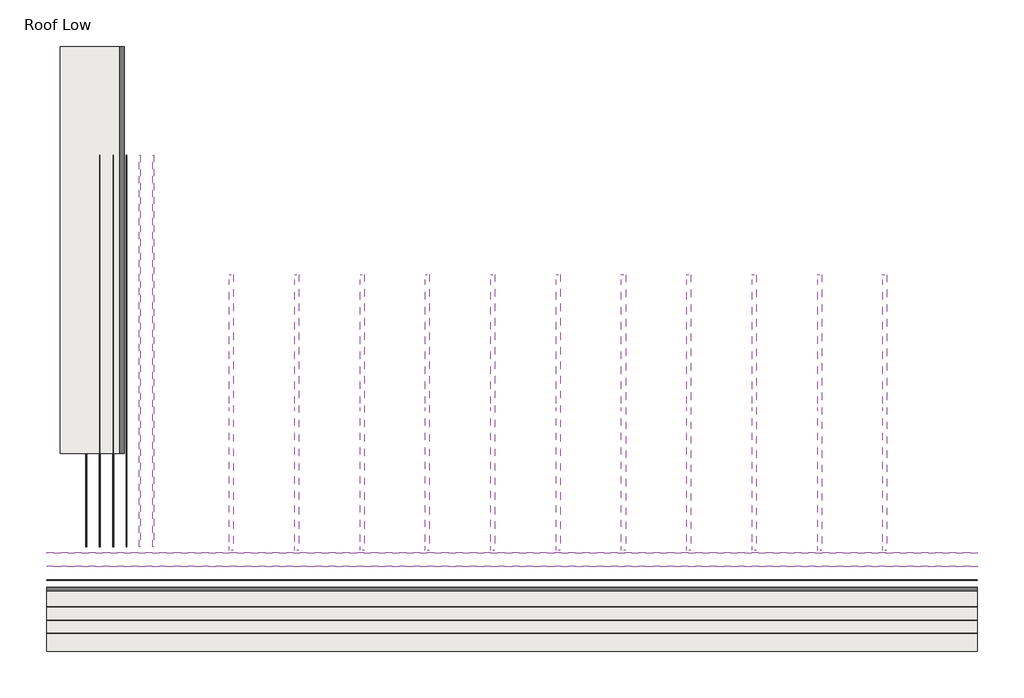
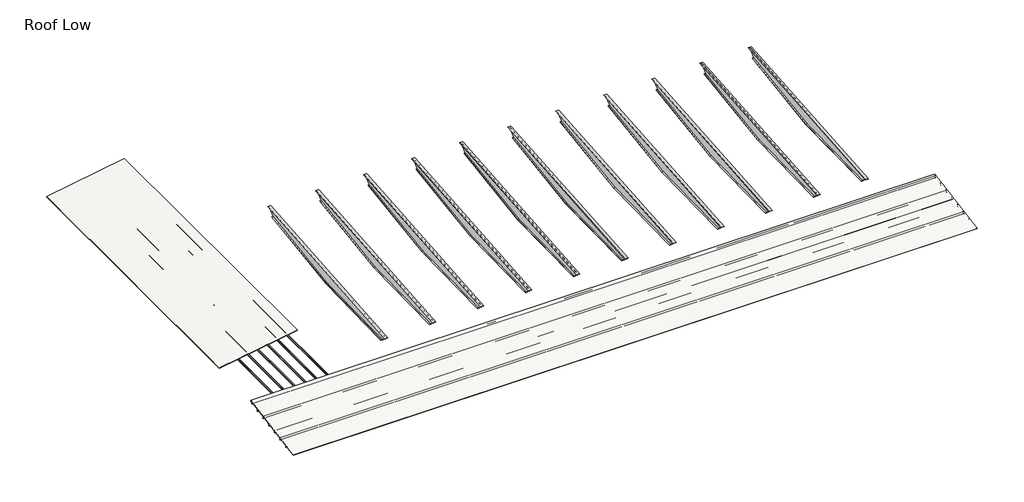
# One storey: 24 beams, 2 roofs.
"""IFC4 building model written with IfcOpenShell, lengths in millimetres."""

import ifcopenshell
import ifcopenshell.guid

model = None  # the IFC model being written
_history = None  # IfcOwnerHistory: only IFC2X3 demands one
_inside = {}  # id of a spatial element -> (the spatial element, [elements in it])
_under = {}  # id of a project, library or spatial element -> (it, [spatial elements below it])
_declared = {}  # id of a project -> (the project, [libraries it declares])
_typed = {}  # id of a type object -> (the type object, [elements of that type])
_made_of = {}  # id of a material, layer set ... -> (it, [elements and type objects made of it])


def new_model(schema):
    """Start an empty IFC model of exactly this schema.

    Asked for "IFC4X3", IfcOpenShell would pick the latest addendum, in which some entities
    have other attributes; the version numbers below select the first issue.
    IFC2X3 requires an IfcOwnerHistory on every rooted entity: one is made here for all.
    """
    global model, _history
    if schema == "IFC4X3":
        model = ifcopenshell.file(schema_version=(4, 3, 0, 0))
    else:
        model = ifcopenshell.file(schema=schema)
    _inside.clear()
    _under.clear()
    _declared.clear()
    _typed.clear()
    _made_of.clear()
    _history = None
    if model.schema == "IFC2X3":
        org = make("IfcOrganization", Name="unknown")
        user = make(
            "IfcPersonAndOrganization",
            ThePerson=make("IfcPerson", FamilyName="unknown"),
            TheOrganization=org,
        )
        app = make(
            "IfcApplication",
            ApplicationDeveloper=org,
            Version="unknown",
            ApplicationFullName="unknown",
            ApplicationIdentifier="unknown",
        )
        _history = make(
            "IfcOwnerHistory",
            OwningUser=user,
            OwningApplication=app,
            ChangeAction="ADDED",
            CreationDate=0,
        )
    return model


def make(cls, **values):
    """One entity of the class cls with the attributes given. An attribute that is None is left unset."""
    return model.create_entity(
        cls, **{name: value for name, value in values.items() if value is not None}
    )


def rooted(cls, **values):
    """An entity with a GlobalId (a new one), such as an element, a storey or a relation."""
    return make(cls, GlobalId=ifcopenshell.guid.new(), OwnerHistory=_history, **values)


def si_unit(unit_type, name, prefix=None):
    """IfcSIUnit, for example si_unit("LENGTHUNIT", "METRE", prefix="MILLI")."""
    return make("IfcSIUnit", UnitType=unit_type, Prefix=prefix, Name=name)


def assignment(units):
    """IfcUnitAssignment: the units of a project."""
    return None if units is None else make("IfcUnitAssignment", Units=units)


def point(xyz):
    """IfcCartesianPoint."""
    return None if xyz is None else make("IfcCartesianPoint", Coordinates=xyz)


def direction(xyz):
    """IfcDirection."""
    return None if xyz is None else make("IfcDirection", DirectionRatios=xyz)


def frame(location, z_axis=None, x_axis=None):
    """IfcAxis2Placement3D, a coordinate frame: its origin and axes. An axis left out is left unset."""
    return make(
        "IfcAxis2Placement3D",
        Location=point(location),
        Axis=direction(z_axis),
        RefDirection=direction(x_axis),
    )


def frame_2d(location, x_axis=None):
    """IfcAxis2Placement2D, a coordinate frame in the plane: its origin and x axis."""
    return make(
        "IfcAxis2Placement2D", Location=point(location), RefDirection=direction(x_axis)
    )


def origin():
    """The frame at (0, 0, 0) with its axes left unset."""
    return frame((0.0, 0.0, 0.0))


def place(relative_to, where):
    """IfcLocalPlacement: puts the frame where relative to a parent placement (None: the world)."""
    return make(
        "IfcLocalPlacement", PlacementRelTo=relative_to, RelativePlacement=where
    )


def context(
    kind, dimensions, precision=None, world=None, true_north=None, identifier=None
):
    """IfcGeometricRepresentationContext, for example the 3D "Model" context."""
    return make(
        "IfcGeometricRepresentationContext",
        ContextIdentifier=identifier,
        ContextType=kind,
        CoordinateSpaceDimension=dimensions,
        Precision=precision,
        WorldCoordinateSystem=world,
        TrueNorth=true_north,
    )


def project(units=None, contexts=None):
    """IfcProject with its units and contexts."""
    return rooted(
        "IfcProject",
        Name="project",
        RepresentationContexts=contexts,
        UnitsInContext=assignment(units),
    )


def spatial(cls, under=None, at=None, **own):
    """A site, building, storey or space (cls), placed at a placement, below another one or the project."""
    s = rooted(cls, ObjectPlacement=at, **own)
    if under is not None:
        _under.setdefault(under.id(), (under, []))[1].append(s)
    return s


def polyline(points):
    """IfcPolyline through the points."""
    return make("IfcPolyline", Points=[point(p) for p in points])


def circle_curve(where, radius):
    """IfcCircle in the frame where."""
    return make("IfcCircle", Position=where, Radius=radius)


def trimmed(basis, trim1, trim2, sense, master):
    """IfcTrimmedCurve: the piece of a basis curve between two trims."""
    return make(
        "IfcTrimmedCurve",
        BasisCurve=basis,
        Trim1=trim1,
        Trim2=trim2,
        SenseAgreement=sense,
        MasterRepresentation=master,
    )


def segment(curve, same_sense, transition):
    """IfcCompositeCurveSegment."""
    return make(
        "IfcCompositeCurveSegment",
        Transition=transition,
        SameSense=same_sense,
        ParentCurve=curve,
    )


def composite_curve(segments, self_intersect=None):
    """IfcCompositeCurve: segments joined end to end."""
    return make("IfcCompositeCurve", Segments=segments, SelfIntersect=self_intersect)


def outline(outer, holes=None, kind="AREA"):
    """IfcArbitraryClosedProfileDef: a profile drawn as a closed curve; with holes, ...WithVoids."""
    if holes is None:
        return make("IfcArbitraryClosedProfileDef", ProfileType=kind, OuterCurve=outer)
    return make(
        "IfcArbitraryProfileDefWithVoids",
        ProfileType=kind,
        OuterCurve=outer,
        InnerCurves=holes,
    )


def extrude(swept, where, along, depth):
    """IfcExtrudedAreaSolid: the profile swept, set in the frame where, extruded along a direction by depth."""
    return make(
        "IfcExtrudedAreaSolid",
        SweptArea=swept,
        Position=where,
        ExtrudedDirection=direction(along),
        Depth=depth,
    )


def shape(context_of_items, identifier, shape_type, items):
    """IfcShapeRepresentation: the items that make up one representation, for example the "Body"."""
    return make(
        "IfcShapeRepresentation",
        ContextOfItems=context_of_items,
        RepresentationIdentifier=identifier,
        RepresentationType=shape_type,
        Items=items,
    )


def source(mapping_origin, context_of_items, identifier, shape_type, items):
    """IfcRepresentationMap: a shape defined once, which mapped items show again and again."""
    return make(
        "IfcRepresentationMap",
        MappingOrigin=mapping_origin,
        MappedRepresentation=shape(context_of_items, identifier, shape_type, items),
    )


def transform(
    local_origin,
    x_axis=None,
    y_axis=None,
    z_axis=None,
    scale=None,
    scale2=None,
    scale3=None,
    uniform=True,
):
    """IfcCartesianTransformationOperator3D, or its non-uniform kind. x_axis, y_axis, z_axis: its Axis1, 2, 3."""
    if uniform:
        return make(
            "IfcCartesianTransformationOperator3D",
            Axis1=direction(x_axis),
            Axis2=direction(y_axis),
            LocalOrigin=point(local_origin),
            Scale=scale,
            Axis3=direction(z_axis),
        )
    return make(
        "IfcCartesianTransformationOperator3DnonUniform",
        Axis1=direction(x_axis),
        Axis2=direction(y_axis),
        LocalOrigin=point(local_origin),
        Scale=scale,
        Axis3=direction(z_axis),
        Scale2=scale2,
        Scale3=scale3,
    )


def mapped(mapping_source, mapping_target):
    """IfcMappedItem: shows the shape of a source again, moved by a transform."""
    return make(
        "IfcMappedItem", MappingSource=mapping_source, MappingTarget=mapping_target
    )


def made_of(thing, what):
    """Note that an element or type object is made of a material, layer set ...; save() writes the relation."""
    if what is not None:
        _made_of.setdefault(what.id(), (what, []))[1].append(thing)
    return thing


def element(
    cls,
    number,
    at=None,
    inside=None,
    cuts=None,
    type_object=None,
    material=None,
    context=None,
    identifier="Body",
    shape_type=None,
    held_by="IfcProductDefinitionShape",
    body=None,
    shapes=None,
    **own,
):
    """One element of the class cls, such as IfcWall. Its Tag is "e" and its number.

    at: its placement. inside: the storey or other place that contains it. cuts: it is an
    opening in that element (IfcRelVoidsElement). A single representation is given by context,
    identifier, shape_type and body (its items); several are given by shapes. held_by: the class
    of the entity that holds the representations. save() writes the other relations.
    """
    e = rooted(cls, Tag="e%d" % number, ObjectPlacement=at, **own)
    if body is not None:
        shapes = [shape(context, identifier, shape_type, body)]
    if shapes is not None:
        e.Representation = make(held_by, Representations=shapes)
    if inside is not None:
        _inside.setdefault(inside.id(), (inside, []))[1].append(e)
    if cuts is not None:
        rooted(
            "IfcRelVoidsElement", RelatingBuildingElement=cuts, RelatedOpeningElement=e
        )
    if type_object is not None:
        _typed.setdefault(type_object.id(), (type_object, []))[1].append(e)
    return made_of(e, material)


def aggregate(whole, parts):
    """IfcRelAggregates: a whole, such as a stair, and the parts it consists of."""
    return rooted("IfcRelAggregates", RelatingObject=whole, RelatedObjects=parts)


def save(model, path):
    """Write the relations noted so far, then the file.

    IfcRelAggregates (storeys below a building ...), IfcRelContainedInSpatialStructure (elements
    in a storey), IfcRelDefinesByType, IfcRelAssociatesMaterial and IfcRelDeclares: one each for
    every whole, place, type object, material and project.
    """
    for whole, parts in _under.values():
        aggregate(whole, parts)
    for where, things in _inside.values():
        rooted(
            "IfcRelContainedInSpatialStructure",
            RelatedElements=things,
            RelatingStructure=where,
        )
    for kind, things in _typed.values():
        rooted("IfcRelDefinesByType", RelatedObjects=things, RelatingType=kind)
    for what, things in _made_of.values():
        rooted("IfcRelAssociatesMaterial", RelatedObjects=things, RelatingMaterial=what)
    for by, libraries in _declared.values():
        rooted("IfcRelDeclares", RelatingContext=by, RelatedDefinitions=libraries)
    model.write(path)


def family7_family7_14774666(model_context):
    return source(origin(), model_context, "Body", "SweptSolid", [
        extrude(outline(polyline([(-914.4, -14659.3825135), (-1828.8, 0.0), (-914.4, 14336.786696), (-31.75, 15508.1028078), (-31.75, -15542.0325135), (-914.4, -14659.3825135)])), frame((0.0, -15.875, 0.0), z_axis=(0.0, 1.0, 0.0), x_axis=(0.0, 0.0, 1.0)), (0.0, 0.0, 1.0), 31.75),
        extrude(outline(polyline([(-914.4, 14336.786696), (-1828.8, 0.0), (-914.4, -14659.3825135), (-948.3280154, -14625.4544981), (-1860.6130939, 0.0222371), (-949.1562421, 14290.6636049), (-914.4, 14336.786696)])), frame((0.0, -228.6, 0.0), z_axis=(0.0, 1.0, 0.0), x_axis=(0.0, 0.0, 1.0)), (0.0, 0.0, 1.0), 457.2),
        extrude(outline(polyline([(-31.75, 15508.1028078), (0.0, 15550.2364809), (0.0, -15573.7825135), (-31.75, -15542.0325135), (-31.75, 15508.1028078)])), frame((0.0, -228.6, 0.0), z_axis=(0.0, 1.0, 0.0), x_axis=(0.0, 0.0, 1.0)), (0.0, 0.0, 1.0), 457.2),
    ])


def beam_6747da0e(model_context):
    return source(origin(), model_context, "Body", "SweptSolid", [
        extrude(outline(composite_curve([segment(polyline([(63.5, 127.0), (75.745104, 112.4068534), (73.6169367, 110.621109), (62.204539, 124.221875), (3.3005807, 124.221875)]), True, "CONTINUOUS"), segment(trimmed(circle_curve(frame_2d((3.3741066, 122.2381931)), 1.9850441), [point((3.3005807, 124.221875))], [point((1.3890625, 122.2381931))], True, "CARTESIAN"), True, "CONTINUOUS"), segment(polyline([(1.3890625, 122.2381931), (1.3890625, -122.2375)]), True, "CONTINUOUS"), segment(trimmed(circle_curve(frame_2d((-3.3734375, -122.2375)), 4.7625), [point((1.3890625, -122.2375))], [point((-3.3734375, -127.0))], False, "CARTESIAN"), True, "CONTINUOUS"), segment(polyline([(-3.3734375, -127.0), (-63.5, -127.0), (-75.745104, -112.4068534), (-73.6169367, -110.621109), (-62.204539, -124.221875), (-3.2694106, -124.221875)]), True, "CONTINUOUS"), segment(trimmed(circle_curve(frame_2d((-3.3748024, -122.2389339)), 1.9857399), [point((-3.2694106, -124.221875))], [point((-1.3890625, -122.2389339))], True, "CARTESIAN"), True, "CONTINUOUS"), segment(polyline([(-1.3890625, -122.2389339), (-1.3890625, 122.2375)]), True, "CONTINUOUS"), segment(trimmed(circle_curve(frame_2d((3.3734375, 122.2375)), 4.7625), [point((-1.3890625, 122.2375))], [point((3.3734375, 127.0))], False, "CARTESIAN"), True, "CONTINUOUS"), segment(polyline([(3.3734375, 127.0), (63.5, 127.0)]), True, "CONTINUOUS")], self_intersect=False)), frame((-52273.2, 0.0, 0.0), z_axis=(1.0, 0.0, 0.0), x_axis=(0.0, 1.0, 0.0)), (0.0, 0.0, 1.0), 104546.4),
    ])


def beam_884d35ae(model_context):
    return source(origin(), model_context, "Body", "SweptSolid", [
        extrude(outline(composite_curve([segment(polyline([(63.5, 127.0), (75.745104, 112.4068534), (73.6169367, 110.621109), (62.204539, 124.221875), (3.3005807, 124.221875)]), True, "CONTINUOUS"), segment(trimmed(circle_curve(frame_2d((3.3741066, 122.2381931)), 1.9850441), [point((3.3005807, 124.221875))], [point((1.3890625, 122.2381931))], True, "CARTESIAN"), True, "CONTINUOUS"), segment(polyline([(1.3890625, 122.2381931), (1.3890625, -122.2375)]), True, "CONTINUOUS"), segment(trimmed(circle_curve(frame_2d((-3.3734375, -122.2375)), 4.7625), [point((1.3890625, -122.2375))], [point((-3.3734375, -127.0))], False, "CARTESIAN"), True, "CONTINUOUS"), segment(polyline([(-3.3734375, -127.0), (-63.5, -127.0), (-75.745104, -112.4068534), (-73.6169367, -110.621109), (-62.204539, -124.221875), (-3.2694106, -124.221875)]), True, "CONTINUOUS"), segment(trimmed(circle_curve(frame_2d((-3.3748024, -122.2389339)), 1.9857399), [point((-3.2694106, -124.221875))], [point((-1.3890625, -122.2389339))], True, "CARTESIAN"), True, "CONTINUOUS"), segment(polyline([(-1.3890625, -122.2389339), (-1.3890625, 122.2375)]), True, "CONTINUOUS"), segment(trimmed(circle_curve(frame_2d((3.3734375, 122.2375)), 4.7625), [point((-1.3890625, 122.2375))], [point((3.3734375, 127.0))], False, "CARTESIAN"), True, "CONTINUOUS"), segment(polyline([(3.3734375, 127.0), (63.5, 127.0)]), True, "CONTINUOUS")], self_intersect=False)), frame((-22098.0, 0.0, 0.0), z_axis=(1.0, 0.0, 0.0), x_axis=(0.0, 1.0, 0.0)), (0.0, 0.0, 1.0), 44025.82),
    ])


model = new_model("IFC4")

# Units and contexts
model_context = context("Model", 3, world=origin())
ifc_project = project(units=[si_unit("LENGTHUNIT", "METRE", prefix="MILLI")], contexts=[model_context])

# Site, building, storey
site = spatial("IfcSite", under=ifc_project)
building = spatial("IfcBuilding", under=site)
storey = spatial("IfcBuildingStorey", under=building, Name="Roof Low", Elevation=3657.6)

# Beams
placement = place(None, origin())
family7_family7_shape = family7_family7_14774666(model_context)
element("IfcBeam", 1, ObjectType="Family7 : Family7", at=placement, inside=storey, context=model_context, shape_type="MappedRepresentation", body=[
    mapped(family7_family7_shape, transform((586368.9117241, -552426.8407337, 9726.0083875), x_axis=(1.32038933737171e-12, 0.9965457582448788, 0.08304547985374926), y_axis=(-1.0, 1.316111794066913e-12, 0.0), z_axis=(0.0, -0.08304547985374934, 0.9965457582448789))),
])
element("IfcBeam", 2, ObjectType="Family7 : Family7", at=placement, inside=storey, context=model_context, shape_type="MappedRepresentation", body=[
    mapped(family7_family7_shape, transform((593709.5117241, -552426.8407337, 9726.0083875), x_axis=(1.3203893373716879e-12, 0.9965457582448789, 0.08304547985374928), y_axis=(-1.0, 1.3161117940668907e-12, 0.0), z_axis=(0.0, -0.08304547985374937, 0.9965457582448789))),
])
element("IfcBeam", 3, ObjectType="Family7 : Family7", at=placement, inside=storey, context=model_context, shape_type="MappedRepresentation", body=[
    mapped(family7_family7_shape, transform((601050.1117241, -552426.8407337, 9726.0083875), x_axis=(1.3203893373716624e-12, 0.9965457582448789, 0.08304547985374897), y_axis=(-1.0, 1.3161117940668655e-12, 0.0), z_axis=(0.0, -0.08304547985374904, 0.9965457582448789))),
])
element("IfcBeam", 4, ObjectType="Family7 : Family7", at=placement, inside=storey, context=model_context, shape_type="MappedRepresentation", body=[
    mapped(family7_family7_shape, transform((608390.7117241, -552426.8407337, 9726.0083875), x_axis=(1.3203893373716398e-12, 0.9965457582448789, 0.0830454798537492), y_axis=(-1.0, 1.3161117940668428e-12, 0.0), z_axis=(0.0, -0.08304547985374928, 0.9965457582448789))),
])
element("IfcBeam", 5, ObjectType="Family7 : Family7", at=placement, inside=storey, context=model_context, shape_type="MappedRepresentation", body=[
    mapped(family7_family7_shape, transform((615731.3117241, -552426.8407337, 9726.0083875), x_axis=(1.3203893373716176e-12, 0.9965457582448789, 0.08304547985374894), y_axis=(-1.0, 1.3161117940668206e-12, 0.0), z_axis=(0.0, -0.08304547985374901, 0.9965457582448789))),
])
element("IfcBeam", 6, ObjectType="Family7 : Family7", at=placement, inside=storey, context=model_context, shape_type="MappedRepresentation", body=[
    mapped(family7_family7_shape, transform((623071.9117241, -552426.8407337, 9726.0083875), x_axis=(1.3203893373715917e-12, 0.9965457582448788, 0.0830454798537492), y_axis=(-1.0, 1.316111794066795e-12, 0.0), z_axis=(0.0, -0.0830454798537493, 0.9965457582448789))),
])
element("IfcBeam", 7, ObjectType="Family7 : Family7", at=placement, inside=storey, context=model_context, shape_type="MappedRepresentation", body=[
    mapped(family7_family7_shape, transform((630412.5117241, -552426.8407337, 9726.0083875), x_axis=(1.3179754628973985e-12, 0.9965457582448789, 0.08304547985374894), y_axis=(-1.0, 1.3137062576986022e-12, 0.0), z_axis=(0.0, -0.08304547985374901, 0.9965457582448789))),
])
element("IfcBeam", 8, ObjectType="Family7 : Family7", at=placement, inside=storey, context=model_context, shape_type="MappedRepresentation", body=[
    mapped(family7_family7_shape, transform((637753.1117241, -552426.8407337, 9726.0083875), x_axis=(1.317975462897376e-12, 0.9965457582448789, 0.08304547985374888), y_axis=(-1.0, 1.3137062576985798e-12, 0.0), z_axis=(0.0, -0.08304547985374897, 0.9965457582448789))),
])
element("IfcBeam", 9, ObjectType="Family7 : Family7", at=placement, inside=storey, context=model_context, shape_type="MappedRepresentation", body=[
    mapped(family7_family7_shape, transform((645093.7117241, -552426.8407337, 9726.0083875), x_axis=(1.3179754628973506e-12, 0.996545758244879, 0.08304547985374865), y_axis=(-1.0, 1.3137062576985543e-12, 0.0), z_axis=(0.0, -0.08304547985374879, 0.9965457582448789))),
])
element("IfcBeam", 10, ObjectType="Family7 : Family7", at=placement, inside=storey, context=model_context, shape_type="MappedRepresentation", body=[
    mapped(family7_family7_shape, transform((652434.3117241, -552426.8407337, 9726.0083875), x_axis=(1.317975462897328e-12, 0.9965457582448788, 0.08304547985374917), y_axis=(-1.0, 1.313706257698532e-12, 0.0), z_axis=(0.0, -0.08304547985374927, 0.9965457582448789))),
])
element("IfcBeam", 11, ObjectType="Family7 : Family7", at=placement, inside=storey, context=model_context, shape_type="MappedRepresentation", body=[
    mapped(family7_family7_shape, transform((659774.9117241, -552426.8407337, 9726.0083875), x_axis=(1.3179754628973058e-12, 0.9965457582448788, 0.08304547985374891), y_axis=(-0.9999999999999999, 1.3137062576985097e-12, 0.0), z_axis=(0.0, -0.083045479853749, 0.9965457582448789))),
])
beam_shape = beam_6747da0e(model_context)
element("IfcBeam", 12, ObjectType="Girt_Z : 10\"D", at=placement, inside=storey, context=model_context, shape_type="MappedRepresentation", body=[
    mapped(beam_shape, transform((617890.3117239, -568231.6177833, 5372.7057404), x_axis=(1.0, 0.0, 0.0), y_axis=(0.0, 0.9863939238321444, 0.16439898730535388), z_axis=(0.0, -0.16439898730535388, 0.9863939238321444))),
])
element("IfcBeam", 13, ObjectType="Girt_Z : 10\"D", at=placement, inside=storey, context=model_context, shape_type="MappedRepresentation", body=[
    mapped(beam_shape, transform((617890.3117239, -569734.8821232, 5122.1616837), x_axis=(1.0, 0.0, 0.0), y_axis=(0.0, 0.9863939238321444, 0.16439898730535388), z_axis=(0.0, -0.16439898730535388, 0.9863939238321444))),
])
element("IfcBeam", 14, ObjectType="Girt_Z : 10\"D", at=placement, inside=storey, context=model_context, shape_type="MappedRepresentation", body=[
    mapped(beam_shape, transform((617890.3117239, -571238.1464631, 4871.6176271), x_axis=(1.0, 0.0, 0.0), y_axis=(0.0, 0.9863939238321444, 0.16439898730535388), z_axis=(0.0, -0.16439898730535388, 0.9863939238321444))),
])
element("IfcBeam", 15, ObjectType="Girt_Z : 10\"D", at=placement, inside=storey, context=model_context, shape_type="MappedRepresentation", body=[
    mapped(beam_shape, transform((617890.3117239, -572741.410803, 4621.0735704), x_axis=(1.0, 0.0, 0.0), y_axis=(0.0, 0.9863939238321444, 0.16439898730535388), z_axis=(0.0, -0.16439898730535388, 0.9863939238321444))),
])
element("IfcBeam", 16, ObjectType="Girt_Z : 10\"D", at=placement, inside=storey, context=model_context, shape_type="MappedRepresentation", body=[
    mapped(beam_shape, transform((617890.3117239, -574244.6751429, 4370.5295137), x_axis=(1.0, 0.0, 0.0), y_axis=(0.0, 0.9863939238321444, 0.16439898730535388), z_axis=(0.0, -0.16439898730535388, 0.9863939238321444))),
])
element("IfcBeam", 17, ObjectType="Girt_Z : 10\"D", at=placement, inside=storey, context=model_context, shape_type="MappedRepresentation", body=[
    mapped(beam_shape, transform((617890.3117239, -575747.9394829, 4119.9854571), x_axis=(1.0, 0.0, 0.0), y_axis=(0.0, 0.9863939238321444, 0.16439898730535388), z_axis=(0.0, -0.16439898730535388, 0.9863939238321444))),
])
element("IfcBeam", 18, ObjectType="Girt_Z : 10\"D", at=placement, inside=storey, context=model_context, shape_type="MappedRepresentation", body=[
    mapped(beam_shape, transform((617890.3117239, -577251.2038228, 3869.4414004), x_axis=(1.0, 0.0, 0.0), y_axis=(0.0, 0.9863939238321444, 0.16439898730535388), z_axis=(0.0, -0.16439898730535388, 0.9863939238321444))),
])
beam_2_shape = beam_884d35ae(model_context)
element("IfcBeam", 19, ObjectType="Girt_Z : 10\"D", at=placement, inside=storey, context=model_context, shape_type="MappedRepresentation", body=[
    mapped(beam_2_shape, transform((577613.4981197, -545593.3413841, 5277.7495395), x_axis=(0.0, -1.0, 0.0), y_axis=(0.986393923832142, 0.0, 0.16439898730536787), z_axis=(-0.16439898730536787, 0.0, 0.986393923832142))),
])
element("IfcBeam", 20, ObjectType="Girt_Z : 10\"D", at=placement, inside=storey, context=model_context, shape_type="MappedRepresentation", body=[
    mapped(beam_2_shape, transform((576110.2337798, -545593.3413841, 5027.2054829), x_axis=(0.0, -1.0, 0.0), y_axis=(0.986393923832142, 0.0, 0.16439898730536787), z_axis=(-0.16439898730536787, 0.0, 0.986393923832142))),
])
element("IfcBeam", 21, ObjectType="Girt_Z : 10\"D", at=placement, inside=storey, context=model_context, shape_type="MappedRepresentation", body=[
    mapped(beam_2_shape, transform((574606.9694399, -545593.3413841, 4776.6614262), x_axis=(0.0, -1.0, 0.0), y_axis=(0.986393923832142, 0.0, 0.16439898730536787), z_axis=(-0.16439898730536787, 0.0, 0.986393923832142))),
])
element("IfcBeam", 22, ObjectType="Girt_Z : 10\"D", at=placement, inside=storey, context=model_context, shape_type="MappedRepresentation", body=[
    mapped(beam_2_shape, transform((573103.7050999, -545593.3413841, 4526.1173696), x_axis=(0.0, -1.0, 0.0), y_axis=(0.986393923832142, 0.0, 0.16439898730536787), z_axis=(-0.16439898730536787, 0.0, 0.986393923832142))),
])
element("IfcBeam", 23, ObjectType="Girt_Z : 10\"D", at=placement, inside=storey, context=model_context, shape_type="MappedRepresentation", body=[
    mapped(beam_2_shape, transform((571600.44076, -545593.3413841, 4275.5733129), x_axis=(0.0, -1.0, 0.0), y_axis=(0.986393923832142, 0.0, 0.16439898730536787), z_axis=(-0.16439898730536787, 0.0, 0.986393923832142))),
])
element("IfcBeam", 24, ObjectType="Girt_Z : 10\"D", at=placement, inside=storey, context=model_context, shape_type="MappedRepresentation", body=[
    mapped(beam_2_shape, transform((570097.1764201, -545593.3413841, 4025.0292563), x_axis=(0.0, -1.0, 0.0), y_axis=(0.986393923832142, 0.0, 0.16439898730536787), z_axis=(-0.16439898730536787, 0.0, 0.986393923832142))),
])

# Roofs
element("IfcRoof", 25, ObjectType="Roof_High", at=placement, inside=storey, context=model_context, shape_type="SweptSolid", body=[
    extrude(outline(polyline([(-579273.7413841, 3738.3546979), (-567945.3413841, 5626.4213646), (-567945.3413841, 5549.1702804), (-579273.7413841, 3661.1036138), (-579273.7413841, 3738.3546979)])), frame((565617.1117239, 0.0, 0.0), z_axis=(1.0, 0.0, 0.0), x_axis=(0.0, 1.0, 0.0)), (0.0, 0.0, 1.0), 104546.4),
])
element("IfcRoof", 26, ObjectType="Roof_High", at=placement, inside=storey, context=model_context, shape_type="SweptSolid", body=[
    extrude(outline(polyline([(5719.5546979, 579028.3117239), (3738.3546979, 567141.1117239), (3661.1036138, 567141.1117239), (5642.3036138, 579028.3117239), (5719.5546979, 579028.3117239)])), frame((0.0, -557023.3413841, 0.0), z_axis=(0.0, 1.0, 0.0), x_axis=(0.0, 0.0, 1.0)), (0.0, 0.0, 1.0), 45720.0),
])

save(model, "model.ifc")

# Revit data of these elements
# Type "Family7 : Family7"
#   Width = 1' - 6"
#   Web_Thickness = 0' - 1 1/4"
#   Length [instance default] = 69' - 10"
#   Depth_Mid [instance default] = 6' - 0"
#   Depth_End = 3' - 0"
#   Angle_Right = 53.00°
#   Angle_Left = 45.00°
# Type "Girt_Z : 10\"D"
#   Web_Thickness = 0' - 0 7/64"
#   Length [instance default] = 10' - 0"
#   Leg_1 = 0' - 2 1/2"
#   Height = 0' - 10"
# Type "Roof_High"
#   Assembly Code = "B1020"
#   built-in parameter 1001600 = 0.25 (stored number, unit not read)
#   Layers, outside or top first: 0' - 3" no material (function 1)
# Elements 1, 2, 3, 4, 5, 6, 7, 8, 9, 10, 11 (IfcBeam, "Family7 : Family7")
#   Phase Created = Phase 1
# Elements 12, 13, 14, 15, 16, 17, 18, 19, 20, 21, 22, 23, 24 (IfcBeam, "Girt_Z : 10\"D")
#   Phase Created = Phase 1
# Element 25 (IfcRoof, "Roof_High")
#   built-in parameter 1001705 = 18.4594 (stored number, unit not read)
#   built-in parameter 1001701 = 0.0114948 (stored number, unit not read)
#   built-in parameter 1001710 = 33615
#   Phase Created = Phase 1
#   Materials on its faces: "Default Roof"
# Element 26 (IfcRoof, "Roof_High")
#   built-in parameter 1001705 = 18.7649 (stored number, unit not read)
#   built-in parameter 1001701 = 0.0114948 (stored number, unit not read)
#   built-in parameter 1001710 = 33615
#   Phase Created = Phase 1
#   Materials on its faces: "Default Roof"
# Materials
#   "Default Roof": class "Miscellaneous", colour RGB 88 101 114, transparency 0
